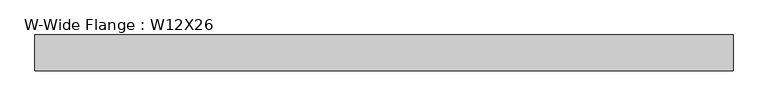
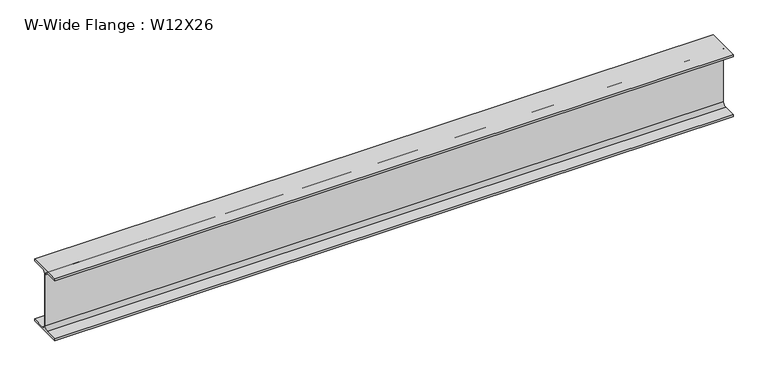
"""IFC4 building model written with IfcOpenShell, lengths in millimetres: beam geometry, W-Wide Flange : W12X26."""

from ifc_helpers import new_model, si_unit, point, frame, frame_2d, origin, place, context, project, spatial, polyline, circle_curve, trimmed, segment, composite_curve, outline, extrude, source, transform, mapped, element, save


def w_wide_flange_w12x26_aed03dbc(model_context):
    return source(origin(), model_context, "Body", "SweptSolid", [
        extrude(outline(composite_curve([segment(polyline([(82.4011719, -145.5539063), (82.4011719, -155.178125), (-82.4011719, -155.178125), (-82.4011719, -145.5539063), (-20.2902344, -145.5539063)]), True, "CONTINUOUS"), segment(trimmed(circle_curve(frame_2d((-20.2902344, -128.190625)), 17.3632812), [point((-20.2902344, -145.5539063))], [point((-2.9269531, -128.190625))], True, "CARTESIAN"), True, "CONTINUOUS"), segment(polyline([(-2.9269531, -128.190625), (-2.9269531, 128.190625)]), True, "CONTINUOUS"), segment(trimmed(circle_curve(frame_2d((-20.2902344, 128.190625)), 17.3632812), [point((-2.9269531, 128.190625))], [point((-20.2902344, 145.5539062))], True, "CARTESIAN"), True, "CONTINUOUS"), segment(polyline([(-20.2902344, 145.5539062), (-82.4011719, 145.5539062), (-82.4011719, 155.178125), (82.4011719, 155.178125), (82.4011719, 145.5539062), (20.2902344, 145.5539062)]), True, "CONTINUOUS"), segment(trimmed(circle_curve(frame_2d((20.2902344, 128.190625)), 17.3632812), [point((20.2902344, 145.5539062))], [point((2.9269531, 128.190625))], True, "CARTESIAN"), True, "CONTINUOUS"), segment(polyline([(2.9269531, 128.190625), (2.9269531, -128.190625)]), True, "CONTINUOUS"), segment(trimmed(circle_curve(frame_2d((20.2902344, -128.190625)), 17.3632812), [point((2.9269531, -128.190625))], [point((20.2902344, -145.5539063))], True, "CARTESIAN"), True, "CONTINUOUS"), segment(polyline([(20.2902344, -145.5539063), (82.4011719, -145.5539063)]), True, "CONTINUOUS")], self_intersect=False)), frame((-1606.5838521, 0.0, 0.0), z_axis=(1.0, 0.0, 0.0), x_axis=(0.0, 1.0, 0.0)), (0.0, 0.0, 1.0), 3213.1677042),
    ])


if __name__ == "__main__":
    model = new_model("IFC4")
    model_context = context("Model", 3, world=origin())
    ifc_project = project(units=[si_unit("LENGTHUNIT", "METRE", prefix="MILLI")], contexts=[model_context])
    site = spatial("IfcSite", under=ifc_project)
    building = spatial("IfcBuilding", under=site)
    placement = place(None, origin())
    w_wide_flange_w12x26_shape = w_wide_flange_w12x26_aed03dbc(model_context)
    element("IfcBeam", 1, ObjectType="W-Wide Flange : W12X26", at=placement, inside=building, context=model_context, shape_type="MappedRepresentation", body=[
        mapped(w_wide_flange_w12x26_shape, transform((0.0, 0.0, 0.0), x_axis=(1.0, 0.0, 0.0), y_axis=(0.0, 1.0, 0.0), z_axis=(0.0, 0.0, 1.0))),
    ])
    save(model, "model.ifc")

# Revit data of these elements
# Type "W-Wide Flange : W12X26"
#   Assembly Code = "B10"
#   W = 26
#   Length [instance default] = 5' - 0"
#   bf = 0' - 6 125/256"
#   d = 1' - 0 7/32"
#   k = 0' - 1 1/16"
#   k2 = 0' - 0 175/256"
#   tf = 0' - 0 97/256"
#   tw = 0' - 0 59/256"
#   A = 0.053125 SF
#   Structural Material [instance default] = none
# Element 1 (IfcBeam, "W-Wide Flange : W12X26")
#   Structural Material = Dark metal
#   Materials on its faces: "Dark metal"
# Materials
#   "Dark metal": class "Generic", colour RGB 44 29 29, transparency 0, Cost = 0
